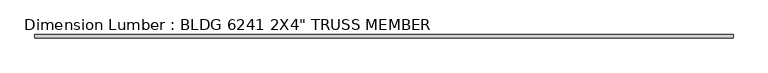
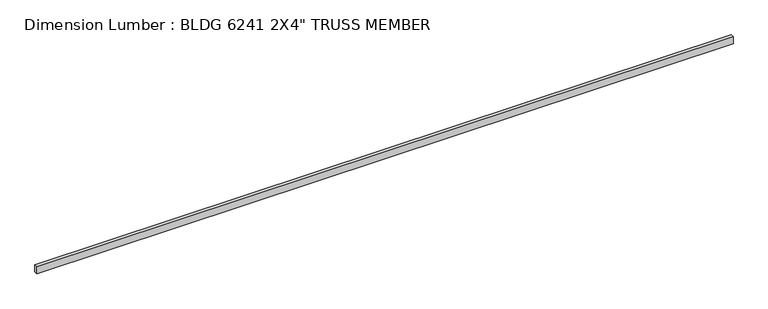
"""IFC4 building model written with IfcOpenShell, lengths in millimetres: beam geometry."""

from ifc_helpers import new_model, si_unit, frame, origin, place, context, project, spatial, polyline, outline, extrude, source, transform, mapped, element, save


def beam_4f005310(model_context):
    return source(origin(), model_context, "Body", "SweptSolid", [
        extrude(outline(polyline([(5035.5499994, 25.4), (5035.5499994, -25.4), (-5035.55, -25.4), (-5035.55, 25.4), (5035.5499994, 25.4)])), frame((0.0, 0.0, -50.8), z_axis=(0.0, 0.0, 1.0), x_axis=(1.0, 0.0, 0.0)), (0.0, 0.0, 1.0), 101.6),
    ])


if __name__ == "__main__":
    model = new_model("IFC4")
    model_context = context("Model", 3, world=origin())
    ifc_project = project(units=[si_unit("LENGTHUNIT", "METRE", prefix="MILLI")], contexts=[model_context])
    site = spatial("IfcSite", under=ifc_project)
    building = spatial("IfcBuilding", under=site)
    placement = place(None, origin())
    beam_shape = beam_4f005310(model_context)
    element("IfcBeam", 1, ObjectType="Dimension Lumber : BLDG 6241 2X4\" TRUSS MEMBER", at=placement, inside=building, context=model_context, shape_type="MappedRepresentation", body=[
        mapped(beam_shape, transform((0.0, 0.0, 0.0), x_axis=(1.0, 0.0, 0.0), y_axis=(0.0, 1.0, 0.0), z_axis=(0.0, 0.0, 1.0))),
    ])
    save(model, "model.ifc")

# Revit data of these elements
# Type "Dimension Lumber : BLDG 6241 2X4\" TRUSS MEMBER"
#   Assembly Code = "B10"
#   A = 0.273472 SF
#   Length [instance default] = 5' - 0"
#   b = 0' - 2"
#   d = 0' - 4"
#   Structural Material [instance default] = Softwood, Lumber
# Element 1 (IfcBeam, "Dimension Lumber : BLDG 6241 2X4\" TRUSS MEMBER")
#   Materials on its faces: "Softwood, Lumber"
# Materials
#   "Softwood, Lumber": class "Wood", colour RGB 223 192 134, transparency 0, Description = "Pinus Echinata", Cost = 0
